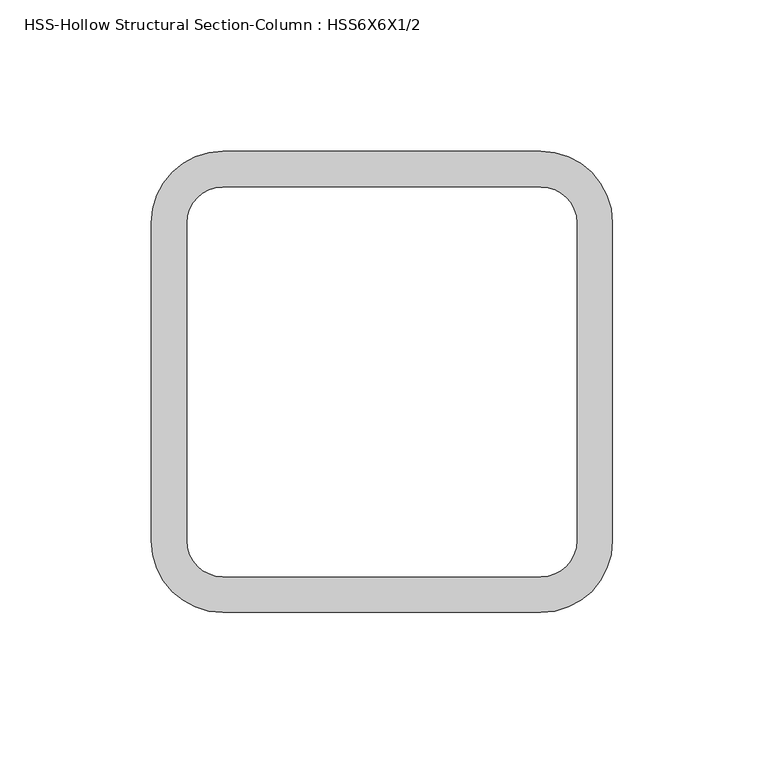
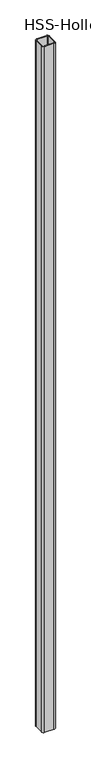
"""IFC4 building model written with IfcOpenShell, lengths in millimetres: column geometry, HSS-Hollow Structural Section-Column : HSS6X6X1/2."""

import ifcopenshell
import ifcopenshell.guid

model = None  # the IFC model being written
_history = None  # IfcOwnerHistory: only IFC2X3 demands one
_inside = {}  # id of a spatial element -> (the spatial element, [elements in it])
_under = {}  # id of a project, library or spatial element -> (it, [spatial elements below it])
_declared = {}  # id of a project -> (the project, [libraries it declares])
_typed = {}  # id of a type object -> (the type object, [elements of that type])
_made_of = {}  # id of a material, layer set ... -> (it, [elements and type objects made of it])


def new_model(schema):
    """Start an empty IFC model of exactly this schema.

    Asked for "IFC4X3", IfcOpenShell would pick the latest addendum, in which some entities
    have other attributes; the version numbers below select the first issue.
    IFC2X3 requires an IfcOwnerHistory on every rooted entity: one is made here for all.
    """
    global model, _history
    if schema == "IFC4X3":
        model = ifcopenshell.file(schema_version=(4, 3, 0, 0))
    else:
        model = ifcopenshell.file(schema=schema)
    _inside.clear()
    _under.clear()
    _declared.clear()
    _typed.clear()
    _made_of.clear()
    _history = None
    if model.schema == "IFC2X3":
        org = make("IfcOrganization", Name="unknown")
        user = make(
            "IfcPersonAndOrganization",
            ThePerson=make("IfcPerson", FamilyName="unknown"),
            TheOrganization=org,
        )
        app = make(
            "IfcApplication",
            ApplicationDeveloper=org,
            Version="unknown",
            ApplicationFullName="unknown",
            ApplicationIdentifier="unknown",
        )
        _history = make(
            "IfcOwnerHistory",
            OwningUser=user,
            OwningApplication=app,
            ChangeAction="ADDED",
            CreationDate=0,
        )
    return model


def make(cls, **values):
    """One entity of the class cls with the attributes given. An attribute that is None is left unset."""
    return model.create_entity(
        cls, **{name: value for name, value in values.items() if value is not None}
    )


def rooted(cls, **values):
    """An entity with a GlobalId (a new one), such as an element, a storey or a relation."""
    return make(cls, GlobalId=ifcopenshell.guid.new(), OwnerHistory=_history, **values)


def si_unit(unit_type, name, prefix=None):
    """IfcSIUnit, for example si_unit("LENGTHUNIT", "METRE", prefix="MILLI")."""
    return make("IfcSIUnit", UnitType=unit_type, Prefix=prefix, Name=name)


def assignment(units):
    """IfcUnitAssignment: the units of a project."""
    return None if units is None else make("IfcUnitAssignment", Units=units)


def point(xyz):
    """IfcCartesianPoint."""
    return None if xyz is None else make("IfcCartesianPoint", Coordinates=xyz)


def direction(xyz):
    """IfcDirection."""
    return None if xyz is None else make("IfcDirection", DirectionRatios=xyz)


def frame(location, z_axis=None, x_axis=None):
    """IfcAxis2Placement3D, a coordinate frame: its origin and axes. An axis left out is left unset."""
    return make(
        "IfcAxis2Placement3D",
        Location=point(location),
        Axis=direction(z_axis),
        RefDirection=direction(x_axis),
    )


def frame_2d(location, x_axis=None):
    """IfcAxis2Placement2D, a coordinate frame in the plane: its origin and x axis."""
    return make(
        "IfcAxis2Placement2D", Location=point(location), RefDirection=direction(x_axis)
    )


def origin():
    """The frame at (0, 0, 0) with its axes left unset."""
    return frame((0.0, 0.0, 0.0))


def place(relative_to, where):
    """IfcLocalPlacement: puts the frame where relative to a parent placement (None: the world)."""
    return make(
        "IfcLocalPlacement", PlacementRelTo=relative_to, RelativePlacement=where
    )


def context(
    kind, dimensions, precision=None, world=None, true_north=None, identifier=None
):
    """IfcGeometricRepresentationContext, for example the 3D "Model" context."""
    return make(
        "IfcGeometricRepresentationContext",
        ContextIdentifier=identifier,
        ContextType=kind,
        CoordinateSpaceDimension=dimensions,
        Precision=precision,
        WorldCoordinateSystem=world,
        TrueNorth=true_north,
    )


def project(units=None, contexts=None):
    """IfcProject with its units and contexts."""
    return rooted(
        "IfcProject",
        Name="project",
        RepresentationContexts=contexts,
        UnitsInContext=assignment(units),
    )


def spatial(cls, under=None, at=None, **own):
    """A site, building, storey or space (cls), placed at a placement, below another one or the project."""
    s = rooted(cls, ObjectPlacement=at, **own)
    if under is not None:
        _under.setdefault(under.id(), (under, []))[1].append(s)
    return s


def polyline(points):
    """IfcPolyline through the points."""
    return make("IfcPolyline", Points=[point(p) for p in points])


def circle_curve(where, radius):
    """IfcCircle in the frame where."""
    return make("IfcCircle", Position=where, Radius=radius)


def trimmed(basis, trim1, trim2, sense, master):
    """IfcTrimmedCurve: the piece of a basis curve between two trims."""
    return make(
        "IfcTrimmedCurve",
        BasisCurve=basis,
        Trim1=trim1,
        Trim2=trim2,
        SenseAgreement=sense,
        MasterRepresentation=master,
    )


def segment(curve, same_sense, transition):
    """IfcCompositeCurveSegment."""
    return make(
        "IfcCompositeCurveSegment",
        Transition=transition,
        SameSense=same_sense,
        ParentCurve=curve,
    )


def composite_curve(segments, self_intersect=None):
    """IfcCompositeCurve: segments joined end to end."""
    return make("IfcCompositeCurve", Segments=segments, SelfIntersect=self_intersect)


def outline(outer, holes=None, kind="AREA"):
    """IfcArbitraryClosedProfileDef: a profile drawn as a closed curve; with holes, ...WithVoids."""
    if holes is None:
        return make("IfcArbitraryClosedProfileDef", ProfileType=kind, OuterCurve=outer)
    return make(
        "IfcArbitraryProfileDefWithVoids",
        ProfileType=kind,
        OuterCurve=outer,
        InnerCurves=holes,
    )


def extrude(swept, where, along, depth):
    """IfcExtrudedAreaSolid: the profile swept, set in the frame where, extruded along a direction by depth."""
    return make(
        "IfcExtrudedAreaSolid",
        SweptArea=swept,
        Position=where,
        ExtrudedDirection=direction(along),
        Depth=depth,
    )


def shape(context_of_items, identifier, shape_type, items):
    """IfcShapeRepresentation: the items that make up one representation, for example the "Body"."""
    return make(
        "IfcShapeRepresentation",
        ContextOfItems=context_of_items,
        RepresentationIdentifier=identifier,
        RepresentationType=shape_type,
        Items=items,
    )


def source(mapping_origin, context_of_items, identifier, shape_type, items):
    """IfcRepresentationMap: a shape defined once, which mapped items show again and again."""
    return make(
        "IfcRepresentationMap",
        MappingOrigin=mapping_origin,
        MappedRepresentation=shape(context_of_items, identifier, shape_type, items),
    )


def transform(
    local_origin,
    x_axis=None,
    y_axis=None,
    z_axis=None,
    scale=None,
    scale2=None,
    scale3=None,
    uniform=True,
):
    """IfcCartesianTransformationOperator3D, or its non-uniform kind. x_axis, y_axis, z_axis: its Axis1, 2, 3."""
    if uniform:
        return make(
            "IfcCartesianTransformationOperator3D",
            Axis1=direction(x_axis),
            Axis2=direction(y_axis),
            LocalOrigin=point(local_origin),
            Scale=scale,
            Axis3=direction(z_axis),
        )
    return make(
        "IfcCartesianTransformationOperator3DnonUniform",
        Axis1=direction(x_axis),
        Axis2=direction(y_axis),
        LocalOrigin=point(local_origin),
        Scale=scale,
        Axis3=direction(z_axis),
        Scale2=scale2,
        Scale3=scale3,
    )


def mapped(mapping_source, mapping_target):
    """IfcMappedItem: shows the shape of a source again, moved by a transform."""
    return make(
        "IfcMappedItem", MappingSource=mapping_source, MappingTarget=mapping_target
    )


def made_of(thing, what):
    """Note that an element or type object is made of a material, layer set ...; save() writes the relation."""
    if what is not None:
        _made_of.setdefault(what.id(), (what, []))[1].append(thing)
    return thing


def element(
    cls,
    number,
    at=None,
    inside=None,
    cuts=None,
    type_object=None,
    material=None,
    context=None,
    identifier="Body",
    shape_type=None,
    held_by="IfcProductDefinitionShape",
    body=None,
    shapes=None,
    **own,
):
    """One element of the class cls, such as IfcWall. Its Tag is "e" and its number.

    at: its placement. inside: the storey or other place that contains it. cuts: it is an
    opening in that element (IfcRelVoidsElement). A single representation is given by context,
    identifier, shape_type and body (its items); several are given by shapes. held_by: the class
    of the entity that holds the representations. save() writes the other relations.
    """
    e = rooted(cls, Tag="e%d" % number, ObjectPlacement=at, **own)
    if body is not None:
        shapes = [shape(context, identifier, shape_type, body)]
    if shapes is not None:
        e.Representation = make(held_by, Representations=shapes)
    if inside is not None:
        _inside.setdefault(inside.id(), (inside, []))[1].append(e)
    if cuts is not None:
        rooted(
            "IfcRelVoidsElement", RelatingBuildingElement=cuts, RelatedOpeningElement=e
        )
    if type_object is not None:
        _typed.setdefault(type_object.id(), (type_object, []))[1].append(e)
    return made_of(e, material)


def aggregate(whole, parts):
    """IfcRelAggregates: a whole, such as a stair, and the parts it consists of."""
    return rooted("IfcRelAggregates", RelatingObject=whole, RelatedObjects=parts)


def save(model, path):
    """Write the relations noted so far, then the file.

    IfcRelAggregates (storeys below a building ...), IfcRelContainedInSpatialStructure (elements
    in a storey), IfcRelDefinesByType, IfcRelAssociatesMaterial and IfcRelDeclares: one each for
    every whole, place, type object, material and project.
    """
    for whole, parts in _under.values():
        aggregate(whole, parts)
    for where, things in _inside.values():
        rooted(
            "IfcRelContainedInSpatialStructure",
            RelatedElements=things,
            RelatingStructure=where,
        )
    for kind, things in _typed.values():
        rooted("IfcRelDefinesByType", RelatedObjects=things, RelatingType=kind)
    for what, things in _made_of.values():
        rooted("IfcRelAssociatesMaterial", RelatedObjects=things, RelatingMaterial=what)
    for by, libraries in _declared.values():
        rooted("IfcRelDeclares", RelatingContext=by, RelatedDefinitions=libraries)
    model.write(path)


def hss_hollow_structural_section_column_hss6x6x1_2_006b3f7d(model_context):
    return source(origin(), model_context, "Body", "SweptSolid", [
        extrude(outline(composite_curve([segment(trimmed(circle_curve(frame_2d((52.578, 52.578)), 23.622), [point((52.578, 76.2))], [point((76.2, 52.578))], False, "CARTESIAN"), True, "CONTINUOUS"), segment(polyline([(76.2, 52.578), (76.2, -52.578)]), True, "CONTINUOUS"), segment(trimmed(circle_curve(frame_2d((52.578, -52.578)), 23.622), [point((76.2, -52.578))], [point((52.578, -76.2))], False, "CARTESIAN"), True, "CONTINUOUS"), segment(polyline([(52.578, -76.2), (-52.578, -76.2)]), True, "CONTINUOUS"), segment(trimmed(circle_curve(frame_2d((-52.578, -52.578)), 23.622), [point((-52.578, -76.2))], [point((-76.2, -52.578))], False, "CARTESIAN"), True, "CONTINUOUS"), segment(polyline([(-76.2, -52.578), (-76.2, 52.578)]), True, "CONTINUOUS"), segment(trimmed(circle_curve(frame_2d((-52.578, 52.578)), 23.622), [point((-76.2, 52.578))], [point((-52.578, 76.2))], False, "CARTESIAN"), True, "CONTINUOUS"), segment(polyline([(-52.578, 76.2), (52.578, 76.2)]), True, "CONTINUOUS")], self_intersect=False), holes=[composite_curve([segment(polyline([(52.578, 64.389), (-52.578, 64.389)]), True, "CONTINUOUS"), segment(trimmed(circle_curve(frame_2d((-52.578, 52.578)), 11.811), [point((-52.578, 64.389))], [point((-64.389, 52.578))], True, "CARTESIAN"), True, "CONTINUOUS"), segment(polyline([(-64.389, 52.578), (-64.389, -52.578)]), True, "CONTINUOUS"), segment(trimmed(circle_curve(frame_2d((-52.578, -52.578)), 11.811), [point((-64.389, -52.578))], [point((-52.578, -64.389))], True, "CARTESIAN"), True, "CONTINUOUS"), segment(polyline([(-52.578, -64.389), (52.578, -64.389)]), True, "CONTINUOUS"), segment(trimmed(circle_curve(frame_2d((52.578, -52.578)), 11.811), [point((52.578, -64.389))], [point((64.389, -52.578))], True, "CARTESIAN"), True, "CONTINUOUS"), segment(polyline([(64.389, -52.578), (64.389, 52.578)]), True, "CONTINUOUS"), segment(trimmed(circle_curve(frame_2d((52.578, 52.578)), 11.811), [point((64.389, 52.578))], [point((52.578, 64.389))], True, "CARTESIAN"), True, "CONTINUOUS")], self_intersect=False)]), frame((0.0, 0.0, 4267.2), z_axis=(0.0, 0.0, 1.0), x_axis=(1.0, 0.0, 0.0)), (0.0, 0.0, 1.0), 8077.2),
    ])


if __name__ == "__main__":
    model = new_model("IFC4")
    model_context = context("Model", 3, world=origin())
    ifc_project = project(units=[si_unit("LENGTHUNIT", "METRE", prefix="MILLI")], contexts=[model_context])
    site = spatial("IfcSite", under=ifc_project)
    building = spatial("IfcBuilding", under=site)
    placement = place(None, origin())
    hss_hollow_structural_section_column_hss6x6x1_2_shape = hss_hollow_structural_section_column_hss6x6x1_2_006b3f7d(model_context)
    element("IfcColumn", 1, ObjectType="HSS-Hollow Structural Section-Column : HSS6X6X1/2", at=placement, inside=building, context=model_context, shape_type="MappedRepresentation", body=[
        mapped(hss_hollow_structural_section_column_hss6x6x1_2_shape, transform((0.0, 0.0, 0.0), x_axis=(1.0, 0.0, 0.0), y_axis=(0.0, 1.0, 0.0), z_axis=(0.0, 0.0, 1.0))),
    ])
    save(model, "model.ifc")

# Revit data of these elements
# Type "HSS-Hollow Structural Section-Column : HSS6X6X1/2"
#   Assembly Code = "B10"
#   Shape = "Square"
#   W = 35.1
#   Ht = 0' - 6"
#   b = 0' - 6"
#   kr = 0' - 0.93"
#   t = 0' - 0.465"
#   A = 0.0676389 SF
#   Structural Material [instance default] = Steel ASTM A500, Grade B, Rectangular and Square
# Element 1 (IfcColumn, "HSS-Hollow Structural Section-Column : HSS6X6X1/2")
#   Materials on its faces: "Steel ASTM A500, Grade B, Rectangular and Square"
# Materials
#   "Steel ASTM A500, Grade B, Rectangular and Square": class "Metal", colour RGB 199 199 199, transparency 0, Description = "Carbon steel", Cost = 0
